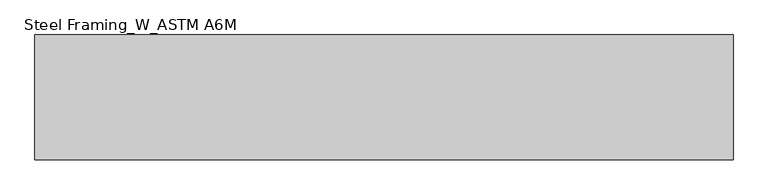
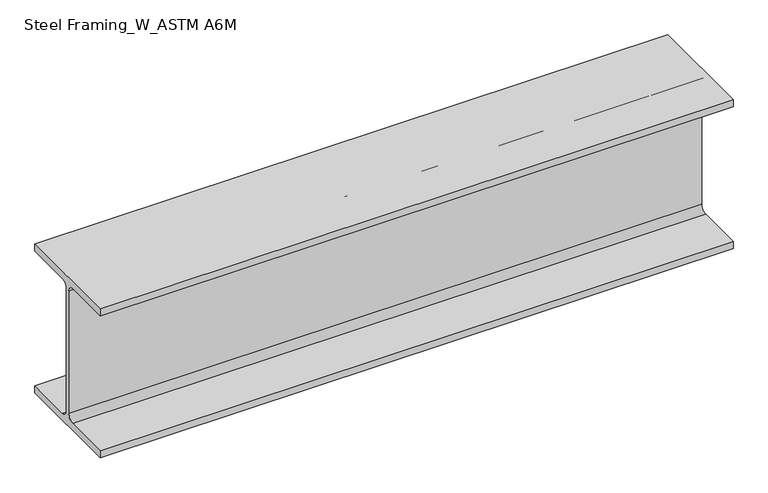
"""IFC4 building model written with IfcOpenShell, lengths in millimetres: beam geometry, Steel Framing_W_ASTM A6M : H_SB_AR_S02_W360x91_B3."""

from ifc_helpers import new_model, si_unit, point, frame, frame_2d, origin, place, context, project, spatial, polyline, circle_curve, trimmed, segment, composite_curve, outline, extrude, source, transform, mapped, element, save


def steel_framing_w_astm_a6m_825bd2fb(model_context):
    return source(origin(), model_context, "Body", "SweptSolid", [
        extrude(outline(composite_curve([segment(polyline([(127.0, -160.1), (127.0, -176.5), (-127.0, -176.5), (-127.0, -160.1), (-19.865, -160.1)]), True, "CONTINUOUS"), segment(trimmed(circle_curve(frame_2d((-19.865, -145.0)), 15.1), [point((-19.865, -160.1))], [point((-4.765, -145.0))], True, "CARTESIAN"), True, "CONTINUOUS"), segment(polyline([(-4.765, -145.0), (-4.765, 145.0)]), True, "CONTINUOUS"), segment(trimmed(circle_curve(frame_2d((-19.865, 145.0)), 15.1), [point((-4.765, 145.0))], [point((-19.865, 160.1))], True, "CARTESIAN"), True, "CONTINUOUS"), segment(polyline([(-19.865, 160.1), (-127.0, 160.1), (-127.0, 176.5), (127.0, 176.5), (127.0, 160.1), (19.865, 160.1)]), True, "CONTINUOUS"), segment(trimmed(circle_curve(frame_2d((19.865, 145.0)), 15.1), [point((19.865, 160.1))], [point((4.765, 145.0))], True, "CARTESIAN"), True, "CONTINUOUS"), segment(polyline([(4.765, 145.0), (4.765, -145.0)]), True, "CONTINUOUS"), segment(trimmed(circle_curve(frame_2d((19.865, -145.0)), 15.1), [point((4.765, -145.0))], [point((19.865, -160.1))], True, "CARTESIAN"), True, "CONTINUOUS"), segment(polyline([(19.865, -160.1), (127.0, -160.1)]), True, "CONTINUOUS")], self_intersect=False)), frame((-710.3, 0.0, 0.0), z_axis=(1.0, 0.0, 0.0), x_axis=(0.0, 1.0, 0.0)), (0.0, 0.0, 1.0), 1420.6),
    ])


if __name__ == "__main__":
    model = new_model("IFC4")
    model_context = context("Model", 3, world=origin())
    ifc_project = project(units=[si_unit("LENGTHUNIT", "METRE", prefix="MILLI")], contexts=[model_context])
    site = spatial("IfcSite", under=ifc_project)
    building = spatial("IfcBuilding", under=site)
    placement = place(None, origin())
    steel_framing_w_astm_a6m_shape = steel_framing_w_astm_a6m_825bd2fb(model_context)
    element("IfcBeam", 1, ObjectType="Steel Framing_W_ASTM A6M : H_SB_AR_S02_W360x91_B3", at=placement, inside=building, context=model_context, shape_type="MappedRepresentation", body=[
        mapped(steel_framing_w_astm_a6m_shape, transform((0.0, 0.0, 0.0), x_axis=(1.0, 0.0, 0.0), y_axis=(0.0, 1.0, 0.0), z_axis=(0.0, 0.0, 1.0))),
    ])
    save(model, "model.ifc")

# Revit data of these elements
# Type "Steel Framing_W_ASTM A6M : H_SB_AR_S02_W360x91_B3"
#   Type Mark = "B3"
#   Section Name Key = "W14x61"
#   Width = 25.4 cm
#   Web Thickness = 0.953 cm
#   Web Fillet = 1.51 cm
#   Warping Constant = 1260000.0 cm⁶
#   Torsional Moment of Inertia = 91.20 cm⁴
#   Section Area = 115.0 cm²
#   Plastic Modulus weak axis = 537.0 cm³
#   Plastic Modulus strong axis = 1670.0 cm³
#   Perimeter = 1.68 m²/m
#   Nominal Weight = 91.00 kgf/m
#   Moment of Inertia weak axis = 4450.00 cm⁴
#   Moment of Inertia strong axis = 26600.00 cm⁴
#   Height = 35.3 cm
#   Flange Thickness = 1.64 cm
#   Elastic Modulus weak axis = 352.0 cm³
#   Elastic Modulus strong axis = 1510.0 cm³
#   Centroid Vertical = 17.65 cm
#   Centroid Horizontal = 12.7 cm
#   Length [instance default] = 1500 mm
#   Structural Material [instance default] = Steel, 45-345
#   Bolt Spacing = 0
#   Assembly Code = ""
# Element 1 (IfcBeam, "Steel Framing_W_ASTM A6M : H_SB_AR_S02_W360x91_B3")
#   Materials on its faces: "Steel, 45-345"
# Materials
#   "Steel, 45-345": class "Metal", colour RGB 189 187 185, transparency 0, Description = "Steel 345 MPa", Cost = 0
